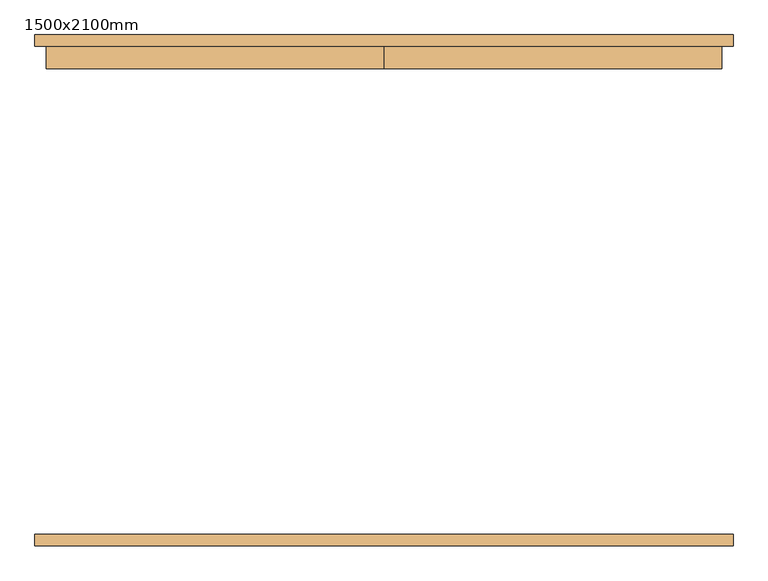
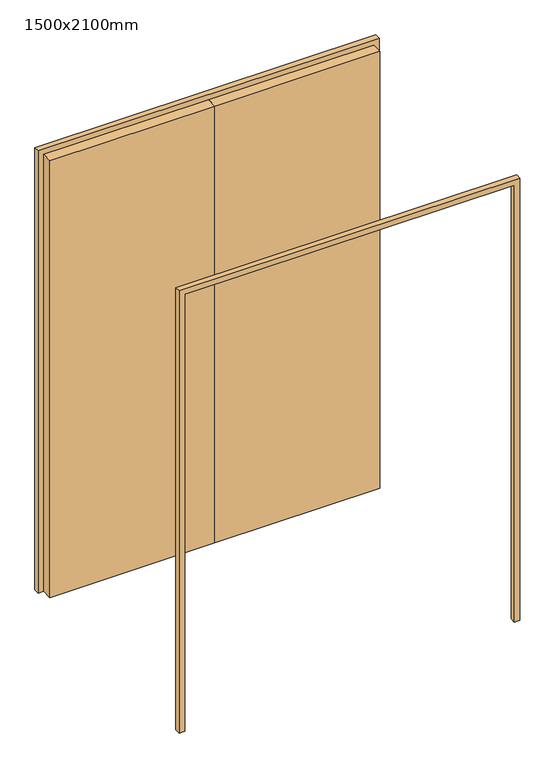
"""IFC4 building model written with IfcOpenShell, lengths in millimetres: door geometry, WWm-DoubleSolid-Flush : 1500x2100mm."""

from ifc_helpers import new_model, si_unit, frame, origin, origin_with_axes, place, context, project, spatial, polyline, outline, extrude, source, transform, mapped, element, save


def door_1500x2100mm_27a640d5(model_context):
    return source(origin(), model_context, "Body", "SweptSolid", [
        extrude(outline(polyline([(0.0, 542.5), (750.0, 542.5), (750.0, 492.5), (0.0, 492.5), (0.0, 542.5)])), origin_with_axes(), (0.0, 0.0, 1.0), 2100.0),
        extrude(outline(polyline([(-750.0, 542.5), (0.0, 542.5), (0.0, 492.5), (-750.0, 492.5), (-750.0, 542.5)])), origin_with_axes(), (0.0, 0.0, 1.0), 2100.0),
        extrude(outline(polyline([(2100.0, -750.0), (2100.0, 750.0), (0.0, 750.0), (0.0, 775.0), (2125.0, 775.0), (2125.0, -775.0), (0.0, -775.0), (0.0, -750.0), (2100.0, -750.0)])), frame((0.0, -567.5, 0.0), z_axis=(0.0, 1.0, 0.0), x_axis=(0.0, 0.0, 1.0)), (0.0, 0.0, 1.0), 25.0),
        extrude(outline(polyline([(2100.0, -750.0), (2100.0, 750.0), (0.0, 750.0), (0.0, 775.0), (2125.0, 775.0), (2125.0, -775.0), (0.0, -775.0), (0.0, -750.0), (2100.0, -750.0)])), frame((0.0, 542.5, 0.0), z_axis=(0.0, 1.0, 0.0), x_axis=(0.0, 0.0, 1.0)), (0.0, 0.0, 1.0), 25.0),
    ])


if __name__ == "__main__":
    model = new_model("IFC4")
    model_context = context("Model", 3, world=origin())
    ifc_project = project(units=[si_unit("LENGTHUNIT", "METRE", prefix="MILLI")], contexts=[model_context])
    site = spatial("IfcSite", under=ifc_project)
    building = spatial("IfcBuilding", under=site)
    placement = place(None, origin())
    door_1500x2100mm_shape = door_1500x2100mm_27a640d5(model_context)
    element("IfcDoor", 1, ObjectType="WWm-DoubleSolid-Flush : 1500x2100mm", at=placement, inside=building, context=model_context, shape_type="MappedRepresentation", body=[
        mapped(door_1500x2100mm_shape, transform((0.0, 0.0, 0.0), x_axis=(1.0, 0.0, 0.0), y_axis=(0.0, 1.0, 0.0), z_axis=(0.0, 0.0, 1.0))),
    ])
    save(model, "model.ifc")

# Revit data of these elements
# Type "WWm-DoubleSolid-Flush : 1500x2100mm"
#   Type Mark = "EX1-56"
#   Construction Type Id = "MDOOR"
#   Assembly Code = "C1020"
#   Analytic Construction = "Metal"
#   Thickness = 50 mm
#   Thermal Resistance (R) = 0.270117 (m²·K)/W
#   Heat Transfer Coefficient (U) = 3.7021 W/(m²·K)
#   Height = 2100 mm
#   Trim Projection Ext = 25 mm
#   Trim Projection Int = 25 mm
#   Trim Width = 25 mm
#   Width = 1500 mm
#   Not 90 Degree [instance default] = no
#   90 Degree [instance default] = yes
#   Door Material = WW-EC-RGB-White
#   Frame Material = WW-EC-RGB-White
#   Visual Light Transmittance = 0
#   Solar Heat Gain Coefficient = 0
#   Function = (empty or 0)
#   Wall Closure = (empty or 0)
# Element 1 (IfcDoor, "WWm-DoubleSolid-Flush : 1500x2100mm")
#   Materials on its faces: "WW-EC-RGB-White"
# Materials
#   "WW-EC-RGB-White": class "Generic", colour RGB 255 255 255, transparency 0, Comments = "If region requests off-white, swith asset color to RGB 231-228-220", Description = "Generic Color", Cost = 0
